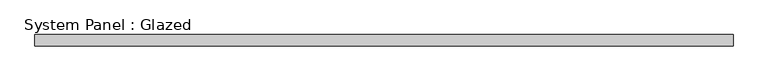
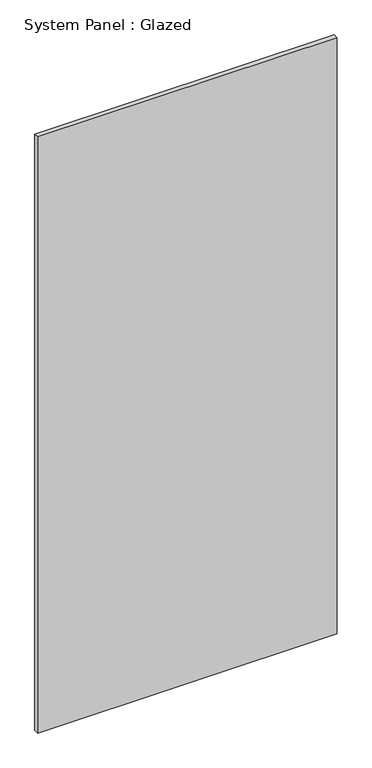
"""IFC4 building model written with IfcOpenShell, lengths in millimetres: plate geometry, System Panel : Glazed."""

import ifcopenshell
import ifcopenshell.guid

model = None  # the IFC model being written
_history = None  # IfcOwnerHistory: only IFC2X3 demands one
_inside = {}  # id of a spatial element -> (the spatial element, [elements in it])
_under = {}  # id of a project, library or spatial element -> (it, [spatial elements below it])
_declared = {}  # id of a project -> (the project, [libraries it declares])
_typed = {}  # id of a type object -> (the type object, [elements of that type])
_made_of = {}  # id of a material, layer set ... -> (it, [elements and type objects made of it])


def new_model(schema):
    """Start an empty IFC model of exactly this schema.

    Asked for "IFC4X3", IfcOpenShell would pick the latest addendum, in which some entities
    have other attributes; the version numbers below select the first issue.
    IFC2X3 requires an IfcOwnerHistory on every rooted entity: one is made here for all.
    """
    global model, _history
    if schema == "IFC4X3":
        model = ifcopenshell.file(schema_version=(4, 3, 0, 0))
    else:
        model = ifcopenshell.file(schema=schema)
    _inside.clear()
    _under.clear()
    _declared.clear()
    _typed.clear()
    _made_of.clear()
    _history = None
    if model.schema == "IFC2X3":
        org = make("IfcOrganization", Name="unknown")
        user = make(
            "IfcPersonAndOrganization",
            ThePerson=make("IfcPerson", FamilyName="unknown"),
            TheOrganization=org,
        )
        app = make(
            "IfcApplication",
            ApplicationDeveloper=org,
            Version="unknown",
            ApplicationFullName="unknown",
            ApplicationIdentifier="unknown",
        )
        _history = make(
            "IfcOwnerHistory",
            OwningUser=user,
            OwningApplication=app,
            ChangeAction="ADDED",
            CreationDate=0,
        )
    return model


def make(cls, **values):
    """One entity of the class cls with the attributes given. An attribute that is None is left unset."""
    return model.create_entity(
        cls, **{name: value for name, value in values.items() if value is not None}
    )


def rooted(cls, **values):
    """An entity with a GlobalId (a new one), such as an element, a storey or a relation."""
    return make(cls, GlobalId=ifcopenshell.guid.new(), OwnerHistory=_history, **values)


def si_unit(unit_type, name, prefix=None):
    """IfcSIUnit, for example si_unit("LENGTHUNIT", "METRE", prefix="MILLI")."""
    return make("IfcSIUnit", UnitType=unit_type, Prefix=prefix, Name=name)


def assignment(units):
    """IfcUnitAssignment: the units of a project."""
    return None if units is None else make("IfcUnitAssignment", Units=units)


def point(xyz):
    """IfcCartesianPoint."""
    return None if xyz is None else make("IfcCartesianPoint", Coordinates=xyz)


def direction(xyz):
    """IfcDirection."""
    return None if xyz is None else make("IfcDirection", DirectionRatios=xyz)


def frame(location, z_axis=None, x_axis=None):
    """IfcAxis2Placement3D, a coordinate frame: its origin and axes. An axis left out is left unset."""
    return make(
        "IfcAxis2Placement3D",
        Location=point(location),
        Axis=direction(z_axis),
        RefDirection=direction(x_axis),
    )


def origin():
    """The frame at (0, 0, 0) with its axes left unset."""
    return frame((0.0, 0.0, 0.0))


def origin_with_axes():
    """The frame at (0, 0, 0) with the z axis (0, 0, 1) and the x axis (1, 0, 0) written out."""
    return frame((0.0, 0.0, 0.0), z_axis=(0.0, 0.0, 1.0), x_axis=(1.0, 0.0, 0.0))


def place(relative_to, where):
    """IfcLocalPlacement: puts the frame where relative to a parent placement (None: the world)."""
    return make(
        "IfcLocalPlacement", PlacementRelTo=relative_to, RelativePlacement=where
    )


def context(
    kind, dimensions, precision=None, world=None, true_north=None, identifier=None
):
    """IfcGeometricRepresentationContext, for example the 3D "Model" context."""
    return make(
        "IfcGeometricRepresentationContext",
        ContextIdentifier=identifier,
        ContextType=kind,
        CoordinateSpaceDimension=dimensions,
        Precision=precision,
        WorldCoordinateSystem=world,
        TrueNorth=true_north,
    )


def project(units=None, contexts=None):
    """IfcProject with its units and contexts."""
    return rooted(
        "IfcProject",
        Name="project",
        RepresentationContexts=contexts,
        UnitsInContext=assignment(units),
    )


def spatial(cls, under=None, at=None, **own):
    """A site, building, storey or space (cls), placed at a placement, below another one or the project."""
    s = rooted(cls, ObjectPlacement=at, **own)
    if under is not None:
        _under.setdefault(under.id(), (under, []))[1].append(s)
    return s


def polyline(points):
    """IfcPolyline through the points."""
    return make("IfcPolyline", Points=[point(p) for p in points])


def outline(outer, holes=None, kind="AREA"):
    """IfcArbitraryClosedProfileDef: a profile drawn as a closed curve; with holes, ...WithVoids."""
    if holes is None:
        return make("IfcArbitraryClosedProfileDef", ProfileType=kind, OuterCurve=outer)
    return make(
        "IfcArbitraryProfileDefWithVoids",
        ProfileType=kind,
        OuterCurve=outer,
        InnerCurves=holes,
    )


def extrude(swept, where, along, depth):
    """IfcExtrudedAreaSolid: the profile swept, set in the frame where, extruded along a direction by depth."""
    return make(
        "IfcExtrudedAreaSolid",
        SweptArea=swept,
        Position=where,
        ExtrudedDirection=direction(along),
        Depth=depth,
    )


def shape(context_of_items, identifier, shape_type, items):
    """IfcShapeRepresentation: the items that make up one representation, for example the "Body"."""
    return make(
        "IfcShapeRepresentation",
        ContextOfItems=context_of_items,
        RepresentationIdentifier=identifier,
        RepresentationType=shape_type,
        Items=items,
    )


def source(mapping_origin, context_of_items, identifier, shape_type, items):
    """IfcRepresentationMap: a shape defined once, which mapped items show again and again."""
    return make(
        "IfcRepresentationMap",
        MappingOrigin=mapping_origin,
        MappedRepresentation=shape(context_of_items, identifier, shape_type, items),
    )


def transform(
    local_origin,
    x_axis=None,
    y_axis=None,
    z_axis=None,
    scale=None,
    scale2=None,
    scale3=None,
    uniform=True,
):
    """IfcCartesianTransformationOperator3D, or its non-uniform kind. x_axis, y_axis, z_axis: its Axis1, 2, 3."""
    if uniform:
        return make(
            "IfcCartesianTransformationOperator3D",
            Axis1=direction(x_axis),
            Axis2=direction(y_axis),
            LocalOrigin=point(local_origin),
            Scale=scale,
            Axis3=direction(z_axis),
        )
    return make(
        "IfcCartesianTransformationOperator3DnonUniform",
        Axis1=direction(x_axis),
        Axis2=direction(y_axis),
        LocalOrigin=point(local_origin),
        Scale=scale,
        Axis3=direction(z_axis),
        Scale2=scale2,
        Scale3=scale3,
    )


def mapped(mapping_source, mapping_target):
    """IfcMappedItem: shows the shape of a source again, moved by a transform."""
    return make(
        "IfcMappedItem", MappingSource=mapping_source, MappingTarget=mapping_target
    )


def made_of(thing, what):
    """Note that an element or type object is made of a material, layer set ...; save() writes the relation."""
    if what is not None:
        _made_of.setdefault(what.id(), (what, []))[1].append(thing)
    return thing


def element(
    cls,
    number,
    at=None,
    inside=None,
    cuts=None,
    type_object=None,
    material=None,
    context=None,
    identifier="Body",
    shape_type=None,
    held_by="IfcProductDefinitionShape",
    body=None,
    shapes=None,
    **own,
):
    """One element of the class cls, such as IfcWall. Its Tag is "e" and its number.

    at: its placement. inside: the storey or other place that contains it. cuts: it is an
    opening in that element (IfcRelVoidsElement). A single representation is given by context,
    identifier, shape_type and body (its items); several are given by shapes. held_by: the class
    of the entity that holds the representations. save() writes the other relations.
    """
    e = rooted(cls, Tag="e%d" % number, ObjectPlacement=at, **own)
    if body is not None:
        shapes = [shape(context, identifier, shape_type, body)]
    if shapes is not None:
        e.Representation = make(held_by, Representations=shapes)
    if inside is not None:
        _inside.setdefault(inside.id(), (inside, []))[1].append(e)
    if cuts is not None:
        rooted(
            "IfcRelVoidsElement", RelatingBuildingElement=cuts, RelatedOpeningElement=e
        )
    if type_object is not None:
        _typed.setdefault(type_object.id(), (type_object, []))[1].append(e)
    return made_of(e, material)


def aggregate(whole, parts):
    """IfcRelAggregates: a whole, such as a stair, and the parts it consists of."""
    return rooted("IfcRelAggregates", RelatingObject=whole, RelatedObjects=parts)


def save(model, path):
    """Write the relations noted so far, then the file.

    IfcRelAggregates (storeys below a building ...), IfcRelContainedInSpatialStructure (elements
    in a storey), IfcRelDefinesByType, IfcRelAssociatesMaterial and IfcRelDeclares: one each for
    every whole, place, type object, material and project.
    """
    for whole, parts in _under.values():
        aggregate(whole, parts)
    for where, things in _inside.values():
        rooted(
            "IfcRelContainedInSpatialStructure",
            RelatedElements=things,
            RelatingStructure=where,
        )
    for kind, things in _typed.values():
        rooted("IfcRelDefinesByType", RelatedObjects=things, RelatingType=kind)
    for what, things in _made_of.values():
        rooted("IfcRelAssociatesMaterial", RelatedObjects=things, RelatingMaterial=what)
    for by, libraries in _declared.values():
        rooted("IfcRelDeclares", RelatingContext=by, RelatedDefinitions=libraries)
    model.write(path)


def system_panel_glazed_3dc34c55(model_context):
    return source(origin(), model_context, "Body", "SweptSolid", [
        extrude(outline(polyline([(796.9250048, 19.05), (-796.9250048, 19.05), (-796.9250048, 44.45), (796.9250048, 44.45), (796.9250048, 19.05)])), origin_with_axes(), (0.0, 0.0, 1.0), 3352.8),
    ])


if __name__ == "__main__":
    model = new_model("IFC4")
    model_context = context("Model", 3, world=origin())
    ifc_project = project(units=[si_unit("LENGTHUNIT", "METRE", prefix="MILLI")], contexts=[model_context])
    site = spatial("IfcSite", under=ifc_project)
    building = spatial("IfcBuilding", under=site)
    placement = place(None, origin())
    system_panel_glazed_shape = system_panel_glazed_3dc34c55(model_context)
    element("IfcPlate", 1, ObjectType="System Panel : Glazed", at=placement, inside=building, context=model_context, shape_type="MappedRepresentation", body=[
        mapped(system_panel_glazed_shape, transform((0.0, 0.0, 0.0), x_axis=(1.0, 0.0, 0.0), y_axis=(0.0, 1.0, 0.0), z_axis=(0.0, 0.0, 1.0))),
    ])
    save(model, "model.ifc")

# Revit data of these elements
# Type "System Panel : Glazed"
#   Construction Type Id = "GSP4R"
#   Analytic Construction = "1/8 in Pilkington single glazing"
#   Visual Light Transmittance = 0.9
#   Solar Heat Gain Coefficient = 0.86
#   Heat Transfer Coefficient (U) = 1.18115 BTU/(h·ft²·°F)
#   Define Thermal Properties by = 1
# Element 1 (IfcPlate, "System Panel : Glazed")
#   Materials on its faces: "Glass"
# Materials
#   "Glass": class "Glass", colour RGB 0 128 192, transparency 0.75, Description = "Soda Lime Glass", Cost = 0
